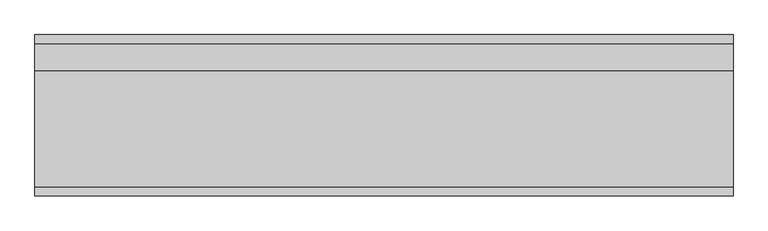
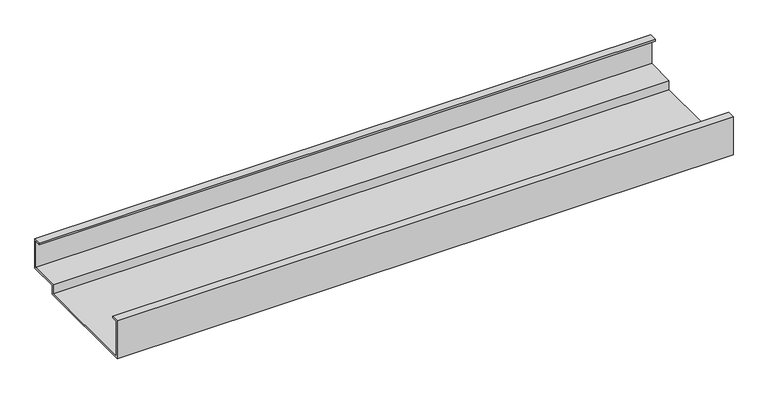
"""IFC4 building model written with IfcOpenShell, lengths in millimetres: proxy geometry, Generic Models 7:Generic Models 1:337419:Generic Models 1:337419 : Generic Models 7:Generic Models 1:337419:13 : Generic Models 7:Generic Models 1:337419:Generic Models 1:337419 : Generic Models 7:Generic Models 1:337419:301336."""

import ifcopenshell
import ifcopenshell.guid

model = None  # the IFC model being written
_history = None  # IfcOwnerHistory: only IFC2X3 demands one
_inside = {}  # id of a spatial element -> (the spatial element, [elements in it])
_under = {}  # id of a project, library or spatial element -> (it, [spatial elements below it])
_declared = {}  # id of a project -> (the project, [libraries it declares])
_typed = {}  # id of a type object -> (the type object, [elements of that type])
_made_of = {}  # id of a material, layer set ... -> (it, [elements and type objects made of it])


def new_model(schema):
    """Start an empty IFC model of exactly this schema.

    Asked for "IFC4X3", IfcOpenShell would pick the latest addendum, in which some entities
    have other attributes; the version numbers below select the first issue.
    IFC2X3 requires an IfcOwnerHistory on every rooted entity: one is made here for all.
    """
    global model, _history
    if schema == "IFC4X3":
        model = ifcopenshell.file(schema_version=(4, 3, 0, 0))
    else:
        model = ifcopenshell.file(schema=schema)
    _inside.clear()
    _under.clear()
    _declared.clear()
    _typed.clear()
    _made_of.clear()
    _history = None
    if model.schema == "IFC2X3":
        org = make("IfcOrganization", Name="unknown")
        user = make(
            "IfcPersonAndOrganization",
            ThePerson=make("IfcPerson", FamilyName="unknown"),
            TheOrganization=org,
        )
        app = make(
            "IfcApplication",
            ApplicationDeveloper=org,
            Version="unknown",
            ApplicationFullName="unknown",
            ApplicationIdentifier="unknown",
        )
        _history = make(
            "IfcOwnerHistory",
            OwningUser=user,
            OwningApplication=app,
            ChangeAction="ADDED",
            CreationDate=0,
        )
    return model


def make(cls, **values):
    """One entity of the class cls with the attributes given. An attribute that is None is left unset."""
    return model.create_entity(
        cls, **{name: value for name, value in values.items() if value is not None}
    )


def rooted(cls, **values):
    """An entity with a GlobalId (a new one), such as an element, a storey or a relation."""
    return make(cls, GlobalId=ifcopenshell.guid.new(), OwnerHistory=_history, **values)


def si_unit(unit_type, name, prefix=None):
    """IfcSIUnit, for example si_unit("LENGTHUNIT", "METRE", prefix="MILLI")."""
    return make("IfcSIUnit", UnitType=unit_type, Prefix=prefix, Name=name)


def assignment(units):
    """IfcUnitAssignment: the units of a project."""
    return None if units is None else make("IfcUnitAssignment", Units=units)


def point(xyz):
    """IfcCartesianPoint."""
    return None if xyz is None else make("IfcCartesianPoint", Coordinates=xyz)


def direction(xyz):
    """IfcDirection."""
    return None if xyz is None else make("IfcDirection", DirectionRatios=xyz)


def frame(location, z_axis=None, x_axis=None):
    """IfcAxis2Placement3D, a coordinate frame: its origin and axes. An axis left out is left unset."""
    return make(
        "IfcAxis2Placement3D",
        Location=point(location),
        Axis=direction(z_axis),
        RefDirection=direction(x_axis),
    )


def origin():
    """The frame at (0, 0, 0) with its axes left unset."""
    return frame((0.0, 0.0, 0.0))


def place(relative_to, where):
    """IfcLocalPlacement: puts the frame where relative to a parent placement (None: the world)."""
    return make(
        "IfcLocalPlacement", PlacementRelTo=relative_to, RelativePlacement=where
    )


def context(
    kind, dimensions, precision=None, world=None, true_north=None, identifier=None
):
    """IfcGeometricRepresentationContext, for example the 3D "Model" context."""
    return make(
        "IfcGeometricRepresentationContext",
        ContextIdentifier=identifier,
        ContextType=kind,
        CoordinateSpaceDimension=dimensions,
        Precision=precision,
        WorldCoordinateSystem=world,
        TrueNorth=true_north,
    )


def project(units=None, contexts=None):
    """IfcProject with its units and contexts."""
    return rooted(
        "IfcProject",
        Name="project",
        RepresentationContexts=contexts,
        UnitsInContext=assignment(units),
    )


def spatial(cls, under=None, at=None, **own):
    """A site, building, storey or space (cls), placed at a placement, below another one or the project."""
    s = rooted(cls, ObjectPlacement=at, **own)
    if under is not None:
        _under.setdefault(under.id(), (under, []))[1].append(s)
    return s


def polyline(points):
    """IfcPolyline through the points."""
    return make("IfcPolyline", Points=[point(p) for p in points])


def outline(outer, holes=None, kind="AREA"):
    """IfcArbitraryClosedProfileDef: a profile drawn as a closed curve; with holes, ...WithVoids."""
    if holes is None:
        return make("IfcArbitraryClosedProfileDef", ProfileType=kind, OuterCurve=outer)
    return make(
        "IfcArbitraryProfileDefWithVoids",
        ProfileType=kind,
        OuterCurve=outer,
        InnerCurves=holes,
    )


def extrude(swept, where, along, depth):
    """IfcExtrudedAreaSolid: the profile swept, set in the frame where, extruded along a direction by depth."""
    return make(
        "IfcExtrudedAreaSolid",
        SweptArea=swept,
        Position=where,
        ExtrudedDirection=direction(along),
        Depth=depth,
    )


def shape(context_of_items, identifier, shape_type, items):
    """IfcShapeRepresentation: the items that make up one representation, for example the "Body"."""
    return make(
        "IfcShapeRepresentation",
        ContextOfItems=context_of_items,
        RepresentationIdentifier=identifier,
        RepresentationType=shape_type,
        Items=items,
    )


def source(mapping_origin, context_of_items, identifier, shape_type, items):
    """IfcRepresentationMap: a shape defined once, which mapped items show again and again."""
    return make(
        "IfcRepresentationMap",
        MappingOrigin=mapping_origin,
        MappedRepresentation=shape(context_of_items, identifier, shape_type, items),
    )


def transform(
    local_origin,
    x_axis=None,
    y_axis=None,
    z_axis=None,
    scale=None,
    scale2=None,
    scale3=None,
    uniform=True,
):
    """IfcCartesianTransformationOperator3D, or its non-uniform kind. x_axis, y_axis, z_axis: its Axis1, 2, 3."""
    if uniform:
        return make(
            "IfcCartesianTransformationOperator3D",
            Axis1=direction(x_axis),
            Axis2=direction(y_axis),
            LocalOrigin=point(local_origin),
            Scale=scale,
            Axis3=direction(z_axis),
        )
    return make(
        "IfcCartesianTransformationOperator3DnonUniform",
        Axis1=direction(x_axis),
        Axis2=direction(y_axis),
        LocalOrigin=point(local_origin),
        Scale=scale,
        Axis3=direction(z_axis),
        Scale2=scale2,
        Scale3=scale3,
    )


def mapped(mapping_source, mapping_target):
    """IfcMappedItem: shows the shape of a source again, moved by a transform."""
    return make(
        "IfcMappedItem", MappingSource=mapping_source, MappingTarget=mapping_target
    )


def made_of(thing, what):
    """Note that an element or type object is made of a material, layer set ...; save() writes the relation."""
    if what is not None:
        _made_of.setdefault(what.id(), (what, []))[1].append(thing)
    return thing


def element(
    cls,
    number,
    at=None,
    inside=None,
    cuts=None,
    type_object=None,
    material=None,
    context=None,
    identifier="Body",
    shape_type=None,
    held_by="IfcProductDefinitionShape",
    body=None,
    shapes=None,
    **own,
):
    """One element of the class cls, such as IfcWall. Its Tag is "e" and its number.

    at: its placement. inside: the storey or other place that contains it. cuts: it is an
    opening in that element (IfcRelVoidsElement). A single representation is given by context,
    identifier, shape_type and body (its items); several are given by shapes. held_by: the class
    of the entity that holds the representations. save() writes the other relations.
    """
    e = rooted(cls, Tag="e%d" % number, ObjectPlacement=at, **own)
    if body is not None:
        shapes = [shape(context, identifier, shape_type, body)]
    if shapes is not None:
        e.Representation = make(held_by, Representations=shapes)
    if inside is not None:
        _inside.setdefault(inside.id(), (inside, []))[1].append(e)
    if cuts is not None:
        rooted(
            "IfcRelVoidsElement", RelatingBuildingElement=cuts, RelatedOpeningElement=e
        )
    if type_object is not None:
        _typed.setdefault(type_object.id(), (type_object, []))[1].append(e)
    return made_of(e, material)


def aggregate(whole, parts):
    """IfcRelAggregates: a whole, such as a stair, and the parts it consists of."""
    return rooted("IfcRelAggregates", RelatingObject=whole, RelatedObjects=parts)


def save(model, path):
    """Write the relations noted so far, then the file.

    IfcRelAggregates (storeys below a building ...), IfcRelContainedInSpatialStructure (elements
    in a storey), IfcRelDefinesByType, IfcRelAssociatesMaterial and IfcRelDeclares: one each for
    every whole, place, type object, material and project.
    """
    for whole, parts in _under.values():
        aggregate(whole, parts)
    for where, things in _inside.values():
        rooted(
            "IfcRelContainedInSpatialStructure",
            RelatedElements=things,
            RelatingStructure=where,
        )
    for kind, things in _typed.values():
        rooted("IfcRelDefinesByType", RelatedObjects=things, RelatingType=kind)
    for what, things in _made_of.values():
        rooted("IfcRelAssociatesMaterial", RelatedObjects=things, RelatingMaterial=what)
    for by, libraries in _declared.values():
        rooted("IfcRelDeclares", RelatingContext=by, RelatedDefinitions=libraries)
    model.write(path)


def generic_models_601f3d41(model_context):
    return source(origin(), model_context, "Body", "SweptSolid", [
        extrude(outline(polyline([(-536557.2913358, 2489.2), (-536557.2913358, 2438.4), (-536606.5038358, 2438.4), (-536606.5038358, 2422.525), (-536792.2413358, 2422.525), (-536792.2413358, 2489.2), (-536779.5413358, 2489.2), (-536779.5413358, 2486.421875), (-536789.4632108, 2486.421875), (-536789.4632108, 2425.303125), (-536609.2819608, 2425.303125), (-536609.2819608, 2441.178125), (-536560.0694608, 2441.178125), (-536560.0694608, 2486.421875), (-536569.9913358, 2486.421875), (-536569.9913358, 2489.2), (-536557.2913358, 2489.2)])), frame((592715.7367242, 0.0, 0.0), z_axis=(1.0, 0.0, 0.0), x_axis=(0.0, 1.0, 0.0)), (0.0, 0.0, 1.0), 1016.0),
    ])


if __name__ == "__main__":
    model = new_model("IFC4")
    model_context = context("Model", 3, world=origin())
    ifc_project = project(units=[si_unit("LENGTHUNIT", "METRE", prefix="MILLI")], contexts=[model_context])
    site = spatial("IfcSite", under=ifc_project)
    building = spatial("IfcBuilding", under=site)
    placement = place(None, origin())
    generic_models_shape = generic_models_601f3d41(model_context)
    element("IfcBuildingElementProxy", 1, Name="Generic Models 7:Generic Models 1:337419:Generic Models 1:337419 : Generic Models 7:Generic Models 1:337419:13 : Generic Models 7:Generic Models 1:337419:Generic Models 1:337419 : Generic Models 7:Generic Models 1:337419:301336", ObjectType="Generic Models 7:Generic Models 1:337419:Generic Models 1:337419 : Generic Models 7:Generic Models 1:337419:13 : Generic Models 7:Generic Models 1:337419:Generic Models 1:337419 : Generic Models 7:Generic Models 1:337419:301336", at=placement, inside=building, context=model_context, shape_type="MappedRepresentation", body=[
        mapped(generic_models_shape, transform((0.0, 0.0, 0.0), x_axis=(1.0, 0.0, 0.0), y_axis=(0.0, 1.0, 0.0), z_axis=(0.0, 0.0, 1.0))),
    ])
    save(model, "model.ifc")

# Revit data of these elements
# Type "Generic Models 7:Generic Models 1:337419:Generic Models 1:337419 : Generic Models 7:Generic Models 1:337419:13 : Generic Models 7:Generic Models 1:337419:Generic Models 1:337419 : Generic Models 7:Generic Models 1:337419:301336"
#   NameOverride = "Generic Models 7:Generic Models 1:337419:Generic Models 1:337419 : Generic Models 7:Generic Models 1:337419:301336"
#   ObjectTypeOverride = "Generic Models 1:337419 : Generic Models 7:Generic Models 1:337419"
#   Reference = "Generic Models 1"
#   Tag = "301336"
# Element 1 (IfcBuildingElementProxy, "Generic Models 7:Generic Models 1:337419:Generic Models 1:337419 : Generic Models 7:Generic Models 1:337419:13 : Generic Models 7:Generic Models 1:337419:Generic Models 1:337419 : Generic Models 7:Generic Models 1:337419:301336")
#   Materials on its faces: "HOLLOW METAL FRAME - SEE DOOR SCHEDULE"
# Materials
#   "HOLLOW METAL FRAME - SEE DOOR SCHEDULE": class "Unassigned", colour RGB 210 209 208, transparency 0, Keynote = "M05121300.02", Cost = 0
